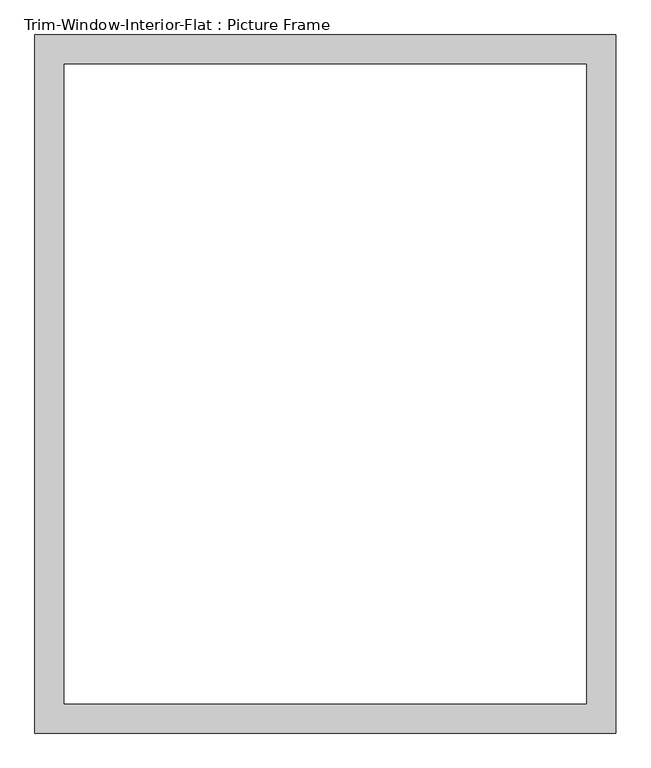
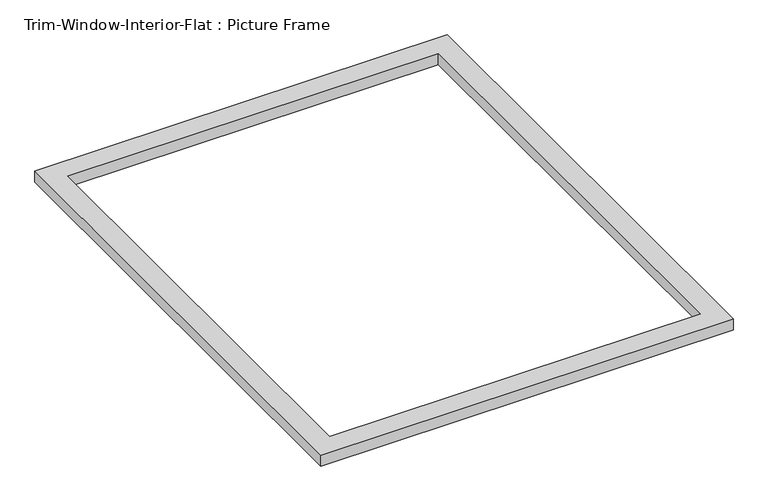
"""IFC4 building model written with IfcOpenShell, lengths in millimetres: proxy geometry, Trim-Window-Interior-Flat : Picture Frame."""

from ifc_helpers import new_model, si_unit, origin, origin_with_axes, place, context, project, spatial, polyline, outline, extrude, source, transform, mapped, element, save


def trim_window_interior_flat_picture_frame_bc4681b1(model_context):
    return source(origin(), model_context, "Body", "SweptSolid", [
        extrude(outline(polyline([(565.15, 44.45), (565.15, -1314.45), (-565.15, -1314.45), (-565.15, 44.45), (565.15, 44.45)]), holes=[polyline([(508.0, -12.7), (-508.0, -12.7), (-508.0, -1257.3), (508.0, -1257.3), (508.0, -12.7)])]), origin_with_axes(), (0.0, 0.0, 1.0), 31.75),
    ])


if __name__ == "__main__":
    model = new_model("IFC4")
    model_context = context("Model", 3, world=origin())
    ifc_project = project(units=[si_unit("LENGTHUNIT", "METRE", prefix="MILLI")], contexts=[model_context])
    site = spatial("IfcSite", under=ifc_project)
    building = spatial("IfcBuilding", under=site)
    placement = place(None, origin())
    trim_window_interior_flat_picture_frame_shape = trim_window_interior_flat_picture_frame_bc4681b1(model_context)
    element("IfcBuildingElementProxy", 1, Name="Trim-Window-Interior-Flat : Picture Frame", ObjectType="Trim-Window-Interior-Flat : Picture Frame", at=placement, inside=building, context=model_context, shape_type="MappedRepresentation", body=[
        mapped(trim_window_interior_flat_picture_frame_shape, transform((0.0, 0.0, 0.0), x_axis=(1.0, 0.0, 0.0), y_axis=(0.0, 1.0, 0.0), z_axis=(0.0, 0.0, 1.0))),
    ])
    save(model, "model.ifc")

# Revit data of these elements
# Type "Trim-Window-Interior-Flat : Picture Frame"
#   Trim Thickness_Picture Frame = 0' - 1 1/4"
#   Trim Width = 0' - 2 1/4"
#   Trim Thickness_with Sill = 0' - 0 3/4"
#   Sill Thickness = 0' - 1 1/4"
#   Opening Width [instance default] = 2' - 0"
#   Opening Height [instance default] = 3' - 0"
#   Default Elevation = 4' - 0"
#   Sill = no
#   Picture Frame = yes
#   Trim Material [instance default] = none
# Element 1 (IfcBuildingElementProxy, "Trim-Window-Interior-Flat : Picture Frame")
#   Opening Width = 3' - 5"
#   Opening Height = 4' - 2"
#   Trim Material = 1X WOOD COMPOSITE TRIM
#   Materials on its faces: "1X WOOD COMPOSITE TRIM"
# Materials
#   "1X WOOD COMPOSITE TRIM": class "Generic", colour RGB 88 61 61, transparency 0, Cost = 0
